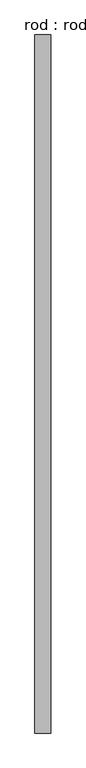
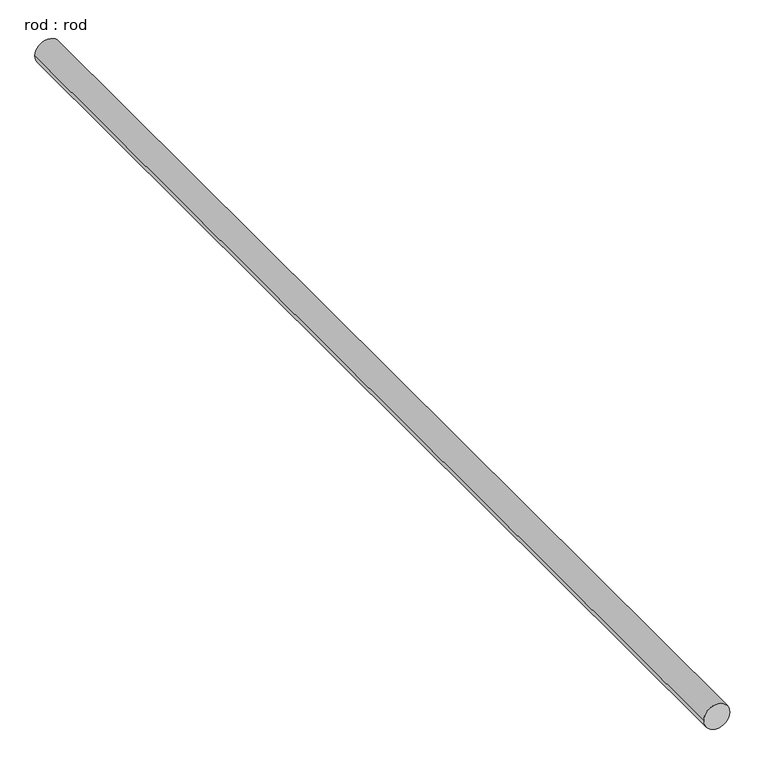
"""IFC4 building model written with IfcOpenShell, lengths in millimetres: proxy geometry, rod : rod."""

from ifc_helpers import new_model, si_unit, point, frame, frame_2d, origin, place, context, project, spatial, circle_curve, trimmed, segment, composite_curve, outline, extrude, source, transform, mapped, element, save


def rod_rod_5451ef31(model_context):
    return source(origin(), model_context, "Body", "SweptSolid", [
        extrude(outline(composite_curve([segment(trimmed(circle_curve(frame_2d((0.0108462, 0.0)), 200.0), [point((0.0108462, 200.0))], [point((0.0108462, -200.0))], False, "CARTESIAN"), True, "CONTINUOUS"), segment(trimmed(circle_curve(frame_2d((0.0108462, 0.0)), 200.0), [point((0.0108462, -200.0))], [point((0.0108462, 200.0))], False, "CARTESIAN"), True, "CONTINUOUS")], self_intersect=False)), frame((0.0, -4768.1859114, 0.0), z_axis=(0.0, 1.0, 0.0), x_axis=(0.0, 0.0, 1.0)), (0.0, 0.0, 1.0), 17721.8290535),
    ])


if __name__ == "__main__":
    model = new_model("IFC4")
    model_context = context("Model", 3, world=origin())
    ifc_project = project(units=[si_unit("LENGTHUNIT", "METRE", prefix="MILLI")], contexts=[model_context])
    site = spatial("IfcSite", under=ifc_project)
    building = spatial("IfcBuilding", under=site)
    placement = place(None, origin())
    rod_rod_shape = rod_rod_5451ef31(model_context)
    element("IfcBuildingElementProxy", 1, Name="rod : rod", ObjectType="rod : rod", at=placement, inside=building, context=model_context, shape_type="MappedRepresentation", body=[
        mapped(rod_rod_shape, transform((0.0, 0.0, 0.0), x_axis=(1.0, 0.0, 0.0), y_axis=(0.0, 1.0, 0.0), z_axis=(0.0, 0.0, 1.0))),
    ])
    save(model, "model.ifc")

# Revit data of these elements
# Type "rod : rod"
#   Default Elevation = 0
